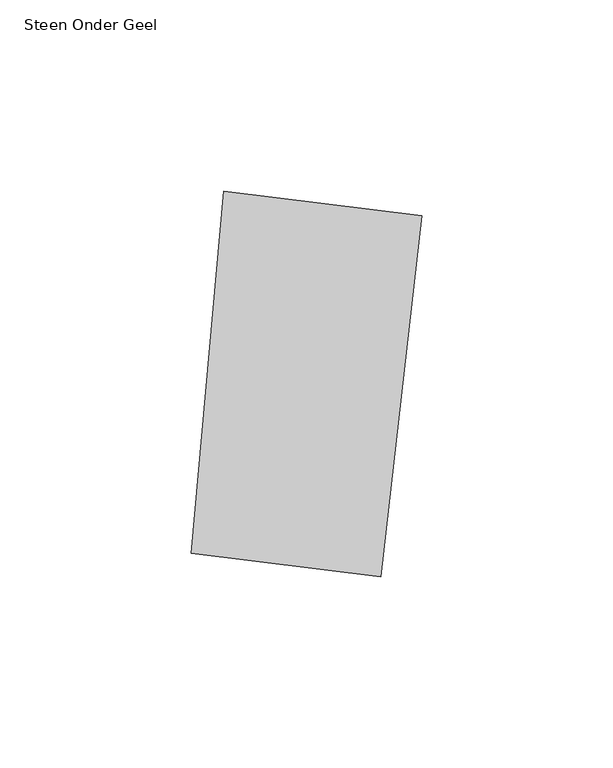
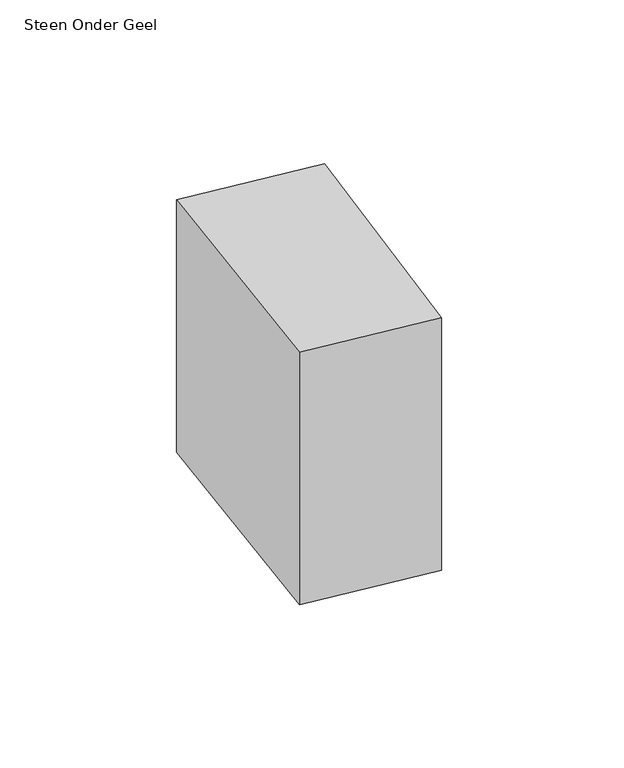
"""IFC4 building model written with IfcOpenShell, lengths in millimetres: proxy geometry, 00_GMA_steen_versie_4 : Steen Onder Geel."""

from ifc_helpers import new_model, si_unit, origin, origin_with_axes, place, context, project, spatial, polyline, outline, extrude, source, transform, mapped, element, save


def steen_onder_geel_edb5e377(model_context):
    return source(origin(), model_context, "Body", "SweptSolid", [
        extrude(outline(polyline([(105.6171528, 113.9316222), (95.0062898, 19.5196518), (45.3842219, 25.6556419), (53.9000965, 120.3287524), (105.6171528, 113.9316222)])), origin_with_axes(), (0.0, 0.0, 1.0), 100.0),
    ])


if __name__ == "__main__":
    model = new_model("IFC4")
    model_context = context("Model", 3, world=origin())
    ifc_project = project(units=[si_unit("LENGTHUNIT", "METRE", prefix="MILLI")], contexts=[model_context])
    site = spatial("IfcSite", under=ifc_project)
    building = spatial("IfcBuilding", under=site)
    placement = place(None, origin())
    steen_onder_geel_shape = steen_onder_geel_edb5e377(model_context)
    element("IfcBuildingElementProxy", 1, Name="00_GMA_steen_versie_4 : Steen Onder Geel", ObjectType="00_GMA_steen_versie_4 : Steen Onder Geel", at=placement, inside=building, context=model_context, shape_type="MappedRepresentation", body=[
        mapped(steen_onder_geel_shape, transform((0.0, 0.0, 0.0), x_axis=(1.0, 0.0, 0.0), y_axis=(0.0, 1.0, 0.0), z_axis=(0.0, 0.0, 1.0))),
    ])
    save(model, "model.ifc")

# Revit data of these elements
# Type "00_GMA_steen_versie_4 : Steen Onder Geel"
#   StootVoegHalfBoven [instance default] = 5 mm
#   StootVoegHalf [instance default] = 5 mm
#   StootVoegBreedteOnder = 10 mm
#   StootVoegBreedteBoven = 10 mm
#   Steendikte = 100 mm
#   LintVoegOnderHalf = 0 mm
#   LintVoegOnder = 0 mm
#   LintVoegBovenHalf = 5 mm
#   LintVoegBoven = 10 mm
#   materiaal = 21_steen_geel
#   MateriaalVoeg = none
#   Default Elevation = 0
# Element 1 (IfcBuildingElementProxy, "00_GMA_steen_versie_4 : Steen Onder Geel")
#   Materials on its faces: "21_steen_geel"
# Materials
#   "21_steen_geel": class "Unassigned", colour RGB 202 202 0, transparency 0, Cost = 0
